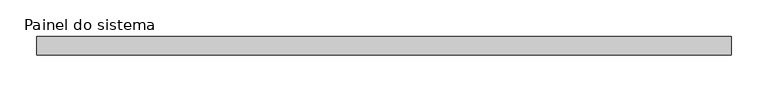
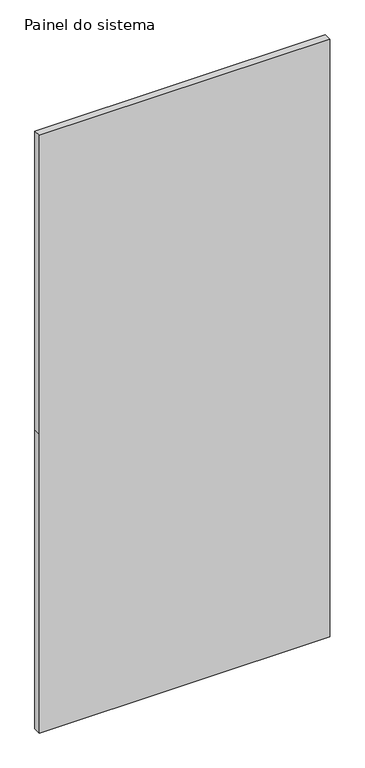
"""IFC4 building model written with IfcOpenShell, lengths in millimetres: plate geometry, Painel do sistema : Envidraçado."""

from ifc_helpers import new_model, si_unit, frame, origin, place, context, project, spatial, polyline, outline, extrude, source, transform, mapped, element, save


def painel_do_sistema_816baa59(model_context):
    return source(origin(), model_context, "Body", "SweptSolid", [
        extrude(outline(polyline([(0.0, -470.855), (0.0, 470.855), (1025.0, 470.855), (2050.0, 470.855), (2050.0, -470.855), (1025.0, -470.855), (0.0, -470.855)])), frame((0.0, -49.5, 0.0), z_axis=(0.0, 1.0, 0.0), x_axis=(0.0, 0.0, 1.0)), (0.0, 0.0, 1.0), 25.0),
    ])


if __name__ == "__main__":
    model = new_model("IFC4")
    model_context = context("Model", 3, world=origin())
    ifc_project = project(units=[si_unit("LENGTHUNIT", "METRE", prefix="MILLI")], contexts=[model_context])
    site = spatial("IfcSite", under=ifc_project)
    building = spatial("IfcBuilding", under=site)
    placement = place(None, origin())
    painel_do_sistema_shape = painel_do_sistema_816baa59(model_context)
    element("IfcPlate", 1, ObjectType="Painel do sistema : Envidraçado", at=placement, inside=building, context=model_context, shape_type="MappedRepresentation", body=[
        mapped(painel_do_sistema_shape, transform((0.0, 0.0, 0.0), x_axis=(1.0, 0.0, 0.0), y_axis=(0.0, 1.0, 0.0), z_axis=(0.0, 0.0, 1.0))),
    ])
    save(model, "model.ifc")

# Revit data of these elements
# Type "Painel do sistema : Envidraçado"
#   Construction Type Id = "GSP4R"
#   Analytic Construction = "Vidraça única Pilkington 1/8 pol"
#   Visual Light Transmittance = 0.9
#   Solar Heat Gain Coefficient = 0.86
#   Heat Transfer Coefficient (U) = 6.7069 W/(m²·K)
# Element 1 (IfcPlate, "Painel do sistema : Envidraçado")
#   Materials on its faces: ".VIDRO GENÉRICO"
# Materials
#   ".VIDRO GENÉRICO": class ".CC_VIDRO", colour RGB 0 128 192, transparency 0.9, Description = "Vidro comum", Cost = 0
